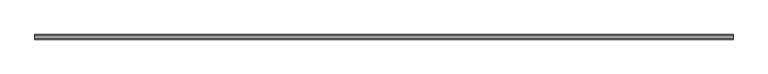
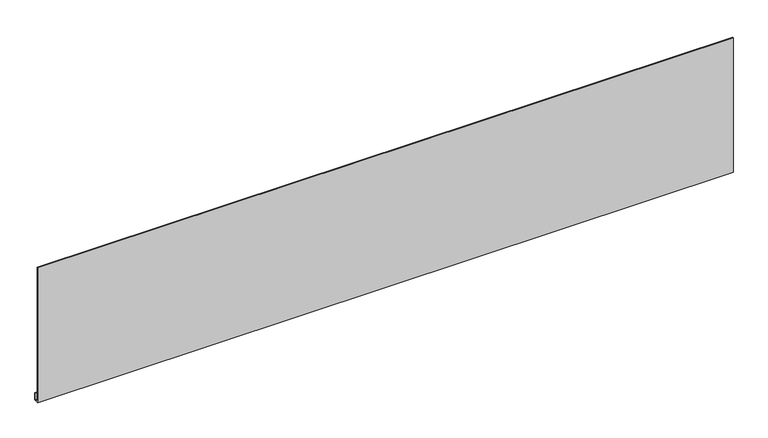
"""IFC4 building model written with IfcOpenShell, lengths in millimetres: proxy geometry, METALFLASHING : METALFLASHING."""

from ifc_helpers import new_model, si_unit, frame, origin, place, context, project, spatial, polyline, outline, extrude, source, transform, mapped, element, save


def generic_models_82097f42(model_context):
    return source(origin(), model_context, "Body", "SweptSolid", [
        extrude(outline(polyline([(-5588.365723, 42324.066406), (-5601.520996, 42324.066406), (-5601.520996, 42733.710938), (-5598.980996, 42733.710938), (-5598.980996, 42326.606406), (-5590.905723, 42326.606406), (-5590.905723, 42345.332031), (-5588.365723, 42345.332031), (-5588.365723, 42324.066406)])), frame((12382.7678845, 0.0, 0.0), z_axis=(1.0, 0.0, 0.0), x_axis=(0.0, 1.0, 0.0)), (0.0, 0.0, 1.0), 2000.25),
    ])


if __name__ == "__main__":
    model = new_model("IFC4")
    model_context = context("Model", 3, world=origin())
    ifc_project = project(units=[si_unit("LENGTHUNIT", "METRE", prefix="MILLI")], contexts=[model_context])
    site = spatial("IfcSite", under=ifc_project)
    building = spatial("IfcBuilding", under=site)
    placement = place(None, origin())
    generic_models_shape = generic_models_82097f42(model_context)
    element("IfcBuildingElementProxy", 1, Name="METALFLASHING : METALFLASHING", ObjectType="METALFLASHING : METALFLASHING", at=placement, inside=building, context=model_context, shape_type="MappedRepresentation", body=[
        mapped(generic_models_shape, transform((0.0, 0.0, 0.0), x_axis=(1.0, 0.0, 0.0), y_axis=(0.0, 1.0, 0.0), z_axis=(0.0, 0.0, 1.0))),
    ])
    save(model, "model.ifc")

# Revit data of these elements
# Type "METALFLASHING : METALFLASHING"
#   NameOverride = "METALFLASHING"
# Element 1 (IfcBuildingElementProxy, "METALFLASHING : METALFLASHING")
#   Materials on its faces: "16 GA. COPPER BRAKE METAL FLASHING"
# Materials
#   "16 GA. COPPER BRAKE METAL FLASHING": class "Unassigned", colour RGB 128 128 128, transparency 0
